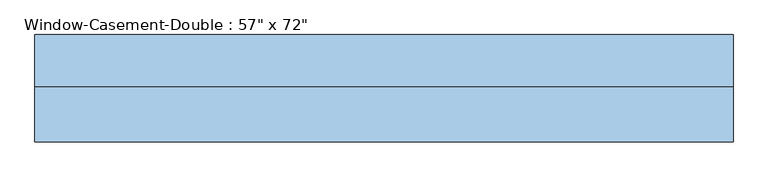
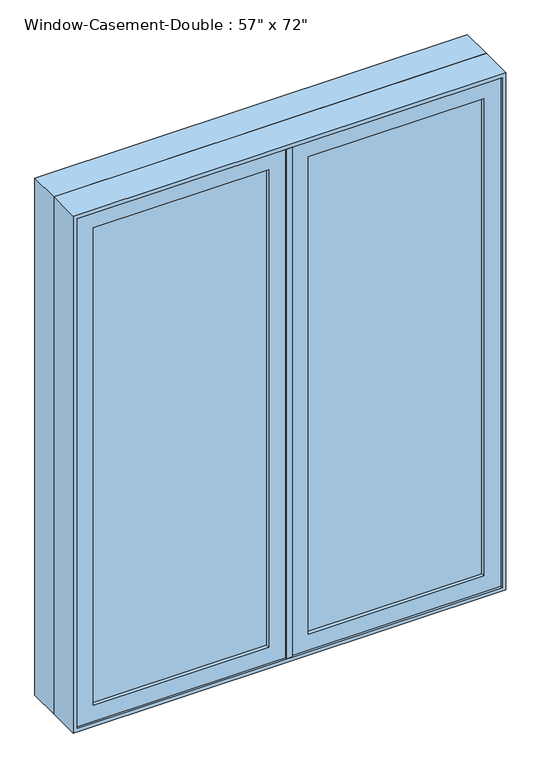
"""IFC4 building model written with IfcOpenShell, lengths in millimetres: window geometry."""

from ifc_helpers import new_model, si_unit, frame, origin, place, context, project, spatial, polyline, outline, extrude, faceted_brep, source, transform, mapped, element, save


def window_525d30cb(model_context):
    return source(origin(), model_context, "Body", "SolidModel", [
        faceted_brep([(9.525, -120.65, 2730.5), (9.525, -69.85, 2730.5), (-9.525, -69.85, 2730.5), (-9.525, -120.65, 2730.5), (9.525, -120.65, 927.1), (-9.525, -120.65, 927.1), (-9.525, -69.85, 927.1), (9.525, -69.85, 927.1), (-9.525, -69.85, 2711.45), (-9.525, -69.85, 946.15), (-30.1625, -69.85, 2711.45), (-30.1625, -69.85, 946.15), (-30.1625, -6.35, 2711.45), (-30.1625, -6.35, 946.15), (30.1625, -6.35, 2711.45), (30.1625, -6.35, 946.15), (30.1625, -69.85, 2711.45), (30.1625, -69.85, 946.15), (9.525, -69.85, 2711.45), (9.525, -69.85, 946.15)], [[[0, 1, 2, 3]], [[4, 5, 6, 7]], [[3, 5, 4, 0]], [[2, 8, 9, 6, 5, 3]], [[8, 10, 11, 9]], [[10, 12, 13, 11]], [[12, 14, 15, 13]], [[14, 16, 17, 15]], [[16, 18, 19, 17]], [[0, 4, 7, 19, 18, 1]], [[8, 2, 1, 18]], [[19, 7, 6, 9]], [[9, 11, 13, 15, 17, 19]], [[18, 16, 14, 12, 10, 8]]]),
        extrude(outline(polyline([(-66.675, -101.6), (-654.05, -101.6), (-654.05, -95.25), (-66.675, -95.25), (-66.675, -101.6)])), frame((0.0, 0.0, 984.25), z_axis=(0.0, 0.0, 1.0), x_axis=(1.0, 0.0, 0.0)), (0.0, 0.0, 1.0), 1689.1),
        extrude(outline(polyline([(-654.05, -82.55), (-66.675, -82.55), (-66.675, -88.9), (-654.05, -88.9), (-654.05, -82.55)])), frame((0.0, 0.0, 984.25), z_axis=(0.0, 0.0, 1.0), x_axis=(1.0, 0.0, 0.0)), (0.0, 0.0, 1.0), 1689.1),
        extrude(outline(polyline([(654.05, -101.6), (66.675, -101.6), (66.675, -95.25), (654.05, -95.25), (654.05, -101.6)])), frame((0.0, 0.0, 984.25), z_axis=(0.0, 0.0, 1.0), x_axis=(1.0, 0.0, 0.0)), (0.0, 0.0, 1.0), 1689.1),
        extrude(outline(polyline([(66.675, -82.55), (654.05, -82.55), (654.05, -88.9), (66.675, -88.9), (66.675, -82.55)])), frame((0.0, 0.0, 984.25), z_axis=(0.0, 0.0, 1.0), x_axis=(1.0, 0.0, 0.0)), (0.0, 0.0, 1.0), 1689.1),
        extrude(outline(polyline([(2730.5, -9.525), (2730.5, -711.2), (927.1, -711.2), (927.1, -9.525), (2730.5, -9.525)]), holes=[polyline([(2673.35, -654.05), (2673.35, -66.675), (984.25, -66.675), (984.25, -654.05), (2673.35, -654.05)])]), frame((0.0, -114.3, 0.0), z_axis=(0.0, 1.0, 0.0), x_axis=(0.0, 0.0, 1.0)), (0.0, 0.0, 1.0), 44.45),
        extrude(outline(polyline([(927.1, 9.525), (927.1, 711.2), (2730.5, 711.2), (2730.5, 9.525), (927.1, 9.525)]), holes=[polyline([(984.25, 654.05), (984.25, 66.675), (2673.35, 66.675), (2673.35, 654.05), (984.25, 654.05)])]), frame((0.0, -114.3, 0.0), z_axis=(0.0, 1.0, 0.0), x_axis=(0.0, 0.0, 1.0)), (0.0, 0.0, 1.0), 44.45),
        extrude(outline(polyline([(2743.2, -723.9), (914.4, -723.9), (914.4, 723.9), (2743.2, 723.9), (2743.2, -723.9)]), holes=[polyline([(2724.15, 704.85), (933.45, 704.85), (933.45, -704.85), (2724.15, -704.85), (2724.15, 704.85)])]), frame((0.0, -6.35, 0.0), z_axis=(0.0, 1.0, 0.0), x_axis=(0.0, 0.0, 1.0)), (0.0, 0.0, 1.0), 107.95),
        faceted_brep([(692.15, -69.85, 2711.45), (-692.15, -69.85, 2711.45), (-692.15, -6.35, 2711.45), (692.15, -6.35, 2711.45), (711.2, -120.65, 2730.5), (-711.2, -120.65, 2730.5), (-711.2, -69.85, 2730.5), (711.2, -69.85, 2730.5), (723.9, -6.35, 2743.2), (-723.9, -6.35, 2743.2), (-723.9, -120.65, 2743.2), (723.9, -120.65, 2743.2), (-692.15, -69.85, 946.15), (-692.15, -6.35, 946.15), (-711.2, -120.65, 927.1), (-711.2, -69.85, 927.1), (-723.9, -6.35, 914.4), (-723.9, -120.65, 914.4), (692.15, -69.85, 946.15), (692.15, -6.35, 946.15), (711.2, -120.65, 927.1), (711.2, -69.85, 927.1), (723.9, -6.35, 914.4), (723.9, -120.65, 914.4)], [[[0, 1, 2, 3]], [[4, 5, 6, 7]], [[8, 9, 10, 11]], [[1, 12, 13, 2]], [[5, 14, 15, 6]], [[9, 16, 17, 10]], [[12, 18, 19, 13]], [[14, 20, 21, 15]], [[16, 22, 23, 17]], [[9, 8, 22, 16], [3, 2, 13, 19]], [[18, 0, 3, 19]], [[7, 6, 15, 21], [1, 0, 18, 12]], [[20, 4, 7, 21]], [[22, 8, 11, 23]], [[11, 10, 17, 23], [5, 4, 20, 14]]]),
    ])


if __name__ == "__main__":
    model = new_model("IFC4")
    model_context = context("Model", 3, world=origin())
    ifc_project = project(units=[si_unit("LENGTHUNIT", "METRE", prefix="MILLI")], contexts=[model_context])
    site = spatial("IfcSite", under=ifc_project)
    building = spatial("IfcBuilding", under=site)
    placement = place(None, origin())
    window_shape = window_525d30cb(model_context)
    element("IfcWindow", 1, ObjectType="Window-Casement-Double : 57\" x 72\"", at=placement, inside=building, context=model_context, shape_type="MappedRepresentation", body=[
        mapped(window_shape, transform((0.0, 0.0, 0.0), x_axis=(1.0, 0.0, 0.0), y_axis=(0.0, 1.0, 0.0), z_axis=(0.0, 0.0, 1.0))),
    ])
    save(model, "model.ifc")

# Revit data of these elements
# Type "Window-Casement-Double : 57\" x 72\""
#   Type Mark = "62"
#   Fire Rating = "0.5h"
#   Assembly Code = "B2020100"
#   Analytic Construction = "Double glazing - domestic"
#   Frame Extension [instance default] = 0' - 0 1/4"
#   Window Inset [instance default] = 0' - 0"
#   Wall Thickness [instance default] = 0' - 6"
#   Interior Wall Closure [instance default] = 0' - 2 1/4"
#   Half Width = 2' - 4 1/2"
#   Visual Light Transmittance = 0.81
#   Thermal Resistance (R) = 1.8146 (h·ft²·°F)/BTU
#   Solar Heat Gain Coefficient = 0.76
#   Rough Width = 4' - 9 1/2"
#   Rough Height = 6' - 0 1/2"
#   Height = 6' - 0"
#   Heat Transfer Coefficient (U) = 0.5511 BTU/(h·ft²·°F)
#   Exterior Wall Closure [instance default] = 0' - 1 1/4"
#   Extension Jamb [instance default] = 0' - 2 1/4"
#   Default Sill Height = 3' - 0"
#   Width = 4' - 9"
#   Define Thermal Properties by = 0
#   Muntin Visibility = yes
#   Interior Trim Visibility [instance default] = yes
#   Exterior Trim Visibility [instance default] = yes
#   Extension Jamb Visibility [instance default] = yes
#   Interior Trim Material = Wood - Stained
#   Muntin Pattern = Muntin Pattern_2x2 : Muntin Pattern_2x2
#   Interior Trim = Trim-Window-Interior-Flat : Picture Frame
#   Interior Frame Material = Wood - Stained
#   Glass Panel Material = Glass
#   Exterior Trim Material = Clad - White
#   Exterior Trim = Trim-Window-Exterior-Flat : with Sill
#   Exterior Frame Material = Clad - White
#   Wall Closure = (empty or 0)
# Element 1 (IfcWindow, "Window-Casement-Double : 57\" x 72\"")
#   Wall Thickness = 0' - 8"
#   Extension Jamb = 0' - 4 1/4"
#   Materials on its faces: "Wood - Stained", "Glass", "Clad - White"
# Materials
#   "Wood - Stained": class "Wood", colour RGB 224 178 126, transparency 0, Cost = 0
#   "Glass": class "Glass", colour RGB 236 240 239, transparency 0.5, Description = "Soda Lime Glass", Cost = 0
#   "Clad - White": class "Wood", colour RGB 216 216 204, transparency 0, Cost = 0
